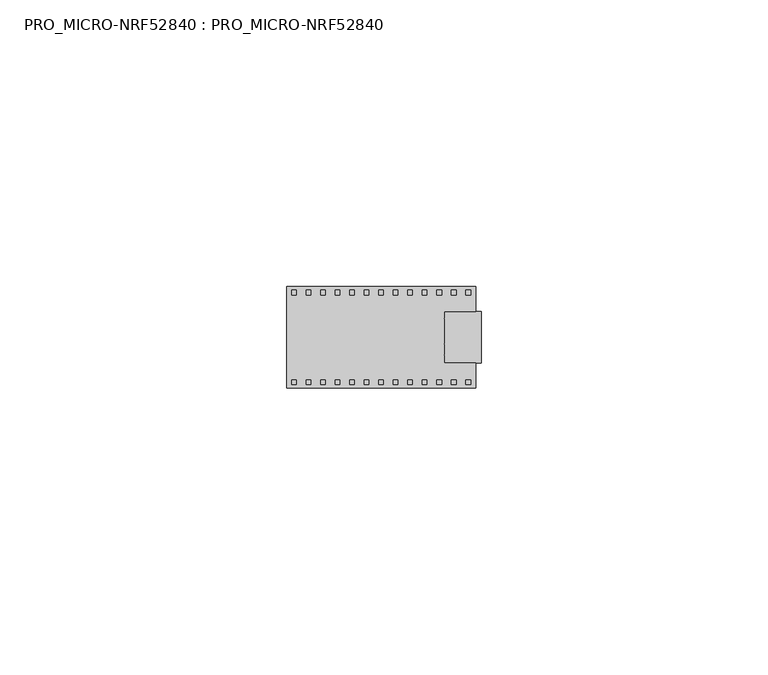
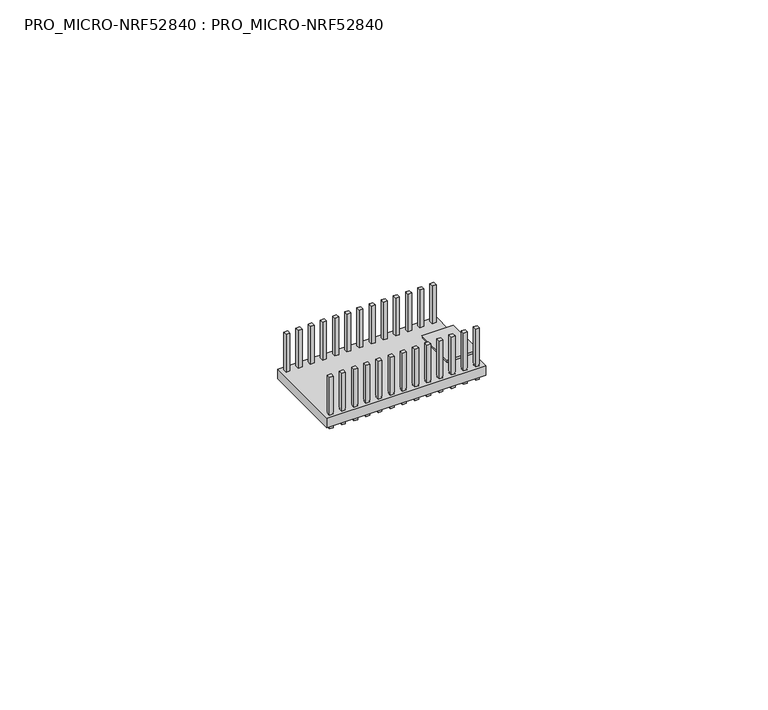
"""IFC4 building model written with IfcOpenShell, lengths in millimetres: furniture geometry, PRO_MICRO-NRF52840 : PRO_MICRO-NRF52840."""

from ifc_helpers import new_model, si_unit, origin, place, context, project, spatial, faceted_brep, source, transform, mapped, element, save


def pro_micro_nrf52840_pro_micro_nrf52840_bcfd0b97(model_context):
    return source(origin(), model_context, "Body", "Brep", [
        faceted_brep([(-14.8, 8.2144911, 11.3), (-15.6, 8.2144911, 11.3), (-15.6, 7.4144911, 11.3), (-14.8, 7.4144911, 11.3), (15.6, 8.2144911, 11.3), (14.8, 8.2144911, 11.3), (14.8, 7.4144911, 11.3), (15.6, 7.4144911, 11.3), (13.0666667, 8.2144911, 11.3), (12.2666667, 8.2144911, 11.3), (12.2666667, 7.4144911, 11.3), (13.0666667, 7.4144911, 11.3), (10.5333333, 8.2144911, 11.3), (9.7333333, 8.2144911, 11.3), (9.7333333, 7.4144911, 11.3), (10.5333333, 7.4144911, 11.3), (8.0, 8.2144911, 11.3), (7.2, 8.2144911, 11.3), (7.2, 7.4144911, 11.3), (8.0, 7.4144911, 11.3), (5.4666667, 8.2144911, 11.3), (4.6666667, 8.2144911, 11.3), (4.6666667, 7.4144911, 11.3), (5.4666667, 7.4144911, 11.3), (2.9333333, 8.2144911, 11.3), (2.1333333, 8.2144911, 11.3), (2.1333333, 7.4144911, 11.3), (2.9333333, 7.4144911, 11.3), (0.4, 8.2144911, 11.3), (-0.4, 8.2144911, 11.3), (-0.4, 7.4144911, 11.3), (0.4, 7.4144911, 11.3), (-2.1333333, 8.2144911, 11.3), (-2.9333333, 8.2144911, 11.3), (-2.9333333, 7.4144911, 11.3), (-2.1333333, 7.4144911, 11.3), (-4.6666667, 8.2144911, 11.3), (-5.4666667, 8.2144911, 11.3), (-5.4666667, 7.4144911, 11.3), (-4.6666667, 7.4144911, 11.3), (-7.2, 8.2144911, 11.3), (-8.0, 8.2144911, 11.3), (-8.0, 7.4144911, 11.3), (-7.2, 7.4144911, 11.3), (-9.7333333, 8.2144911, 11.3), (-10.5333333, 8.2144911, 11.3), (-10.5333333, 7.4144911, 11.3), (-9.7333333, 7.4144911, 11.3), (-12.2666667, 8.2144911, 11.3), (-13.0666667, 8.2144911, 11.3), (-13.0666667, 7.4144911, 11.3), (-12.2666667, 7.4144911, 11.3), (-14.8, 8.2144911, 0.0), (-14.8, 7.4144911, 0.0), (-15.6, 7.4144911, 0.0), (-15.6, 8.2144911, 0.0), (15.6, 8.2144911, 0.0), (15.6, 7.4144911, 0.0), (14.8, 7.4144911, 0.0), (14.8, 8.2144911, 0.0), (13.0666667, 8.2144911, 0.0), (13.0666667, 7.4144911, 0.0), (12.2666667, 7.4144911, 0.0), (12.2666667, 8.2144911, 0.0), (10.5333333, 8.2144911, 0.0), (10.5333333, 7.4144911, 0.0), (9.7333333, 7.4144911, 0.0), (9.7333333, 8.2144911, 0.0), (8.0, 8.2144911, 0.0), (8.0, 7.4144911, 0.0), (7.2, 7.4144911, 0.0), (7.2, 8.2144911, 0.0), (5.4666667, 8.2144911, 0.0), (5.4666667, 7.4144911, 0.0), (4.6666667, 7.4144911, 0.0), (4.6666667, 8.2144911, 0.0), (2.9333333, 8.2144911, 0.0), (2.9333333, 7.4144911, 0.0), (2.1333333, 7.4144911, 0.0), (2.1333333, 8.2144911, 0.0), (0.4, 8.2144911, 0.0), (0.4, 7.4144911, 0.0), (-0.4, 7.4144911, 0.0), (-0.4, 8.2144911, 0.0), (-2.1333333, 8.2144911, 0.0), (-2.1333333, 7.4144911, 0.0), (-2.9333333, 7.4144911, 0.0), (-2.9333333, 8.2144911, 0.0), (-4.6666667, 8.2144911, 0.0), (-4.6666667, 7.4144911, 0.0), (-5.4666667, 7.4144911, 0.0), (-5.4666667, 8.2144911, 0.0), (-7.2, 8.2144911, 0.0), (-7.2, 7.4144911, 0.0), (-8.0, 7.4144911, 0.0), (-8.0, 8.2144911, 0.0), (-9.7333333, 8.2144911, 0.0), (-9.7333333, 7.4144911, 0.0), (-10.5333333, 7.4144911, 0.0), (-10.5333333, 8.2144911, 0.0), (-12.2666667, 8.2144911, 0.0), (-12.2666667, 7.4144911, 0.0), (-13.0666667, 7.4144911, 0.0), (-13.0666667, 8.2144911, 0.0), (-14.8, 8.2144911, 3.0), (-15.6, 8.2144911, 3.0), (-15.6, 8.2144911, 1.0), (-14.8, 8.2144911, 1.0), (-15.6, 7.4144911, 3.0), (-15.6, 7.4144911, 1.0), (-14.8, 7.4144911, 3.0), (-14.8, 7.4144911, 1.0), (15.6, 8.2144911, 3.0), (14.8, 8.2144911, 3.0), (14.8, 8.2144911, 1.0), (15.6, 8.2144911, 1.0), (14.8, 7.4144911, 3.0), (14.8, 7.4144911, 1.0), (15.6, 7.4144911, 3.0), (15.6, 7.4144911, 1.0), (13.0666667, 8.2144911, 3.0), (12.2666667, 8.2144911, 3.0), (12.2666667, 8.2144911, 1.0), (13.0666667, 8.2144911, 1.0), (12.2666667, 7.4144911, 3.0), (12.2666667, 7.4144911, 1.0), (13.0666667, 7.4144911, 3.0), (13.0666667, 7.4144911, 1.0), (10.5333333, 8.2144911, 3.0), (9.7333333, 8.2144911, 3.0), (9.7333333, 8.2144911, 1.0), (10.5333333, 8.2144911, 1.0), (9.7333333, 7.4144911, 3.0), (9.7333333, 7.4144911, 1.0), (10.5333333, 7.4144911, 3.0), (10.5333333, 7.4144911, 1.0), (8.0, 8.2144911, 3.0), (7.2, 8.2144911, 3.0), (7.2, 8.2144911, 1.0), (8.0, 8.2144911, 1.0), (7.2, 7.4144911, 3.0), (7.2, 7.4144911, 1.0), (8.0, 7.4144911, 3.0), (8.0, 7.4144911, 1.0), (5.4666667, 8.2144911, 3.0), (4.6666667, 8.2144911, 3.0), (4.6666667, 8.2144911, 1.0), (5.4666667, 8.2144911, 1.0), (4.6666667, 7.4144911, 3.0), (4.6666667, 7.4144911, 1.0), (5.4666667, 7.4144911, 3.0), (5.4666667, 7.4144911, 1.0), (2.9333333, 8.2144911, 3.0), (2.1333333, 8.2144911, 3.0), (2.1333333, 8.2144911, 1.0), (2.9333333, 8.2144911, 1.0), (2.1333333, 7.4144911, 3.0), (2.1333333, 7.4144911, 1.0), (2.9333333, 7.4144911, 3.0), (2.9333333, 7.4144911, 1.0), (0.4, 8.2144911, 3.0), (-0.4, 8.2144911, 3.0), (-0.4, 8.2144911, 1.0), (0.4, 8.2144911, 1.0), (-0.4, 7.4144911, 3.0), (-0.4, 7.4144911, 1.0), (0.4, 7.4144911, 3.0), (0.4, 7.4144911, 1.0), (-2.1333333, 8.2144911, 3.0), (-2.9333333, 8.2144911, 3.0), (-2.9333333, 8.2144911, 1.0), (-2.1333333, 8.2144911, 1.0), (-2.9333333, 7.4144911, 3.0), (-2.9333333, 7.4144911, 1.0), (-2.1333333, 7.4144911, 3.0), (-2.1333333, 7.4144911, 1.0), (-4.6666667, 8.2144911, 3.0), (-5.4666667, 8.2144911, 3.0), (-5.4666667, 8.2144911, 1.0), (-4.6666667, 8.2144911, 1.0), (-5.4666667, 7.4144911, 3.0), (-5.4666667, 7.4144911, 1.0), (-4.6666667, 7.4144911, 3.0), (-4.6666667, 7.4144911, 1.0), (-7.2, 8.2144911, 3.0), (-8.0, 8.2144911, 3.0), (-8.0, 8.2144911, 1.0), (-7.2, 8.2144911, 1.0), (-8.0, 7.4144911, 3.0), (-8.0, 7.4144911, 1.0), (-7.2, 7.4144911, 3.0), (-7.2, 7.4144911, 1.0), (-9.7333333, 8.2144911, 3.0), (-10.5333333, 8.2144911, 3.0), (-10.5333333, 8.2144911, 1.0), (-9.7333333, 8.2144911, 1.0), (-10.5333333, 7.4144911, 3.0), (-10.5333333, 7.4144911, 1.0), (-9.7333333, 7.4144911, 3.0), (-9.7333333, 7.4144911, 1.0), (-12.2666667, 8.2144911, 3.0), (-13.0666667, 8.2144911, 3.0), (-13.0666667, 8.2144911, 1.0), (-12.2666667, 8.2144911, 1.0), (-13.0666667, 7.4144911, 3.0), (-13.0666667, 7.4144911, 1.0), (-12.2666667, 7.4144911, 3.0), (-12.2666667, 7.4144911, 1.0), (16.5, 8.89, 3.0), (-16.5, 8.89, 3.0), (-16.5, -8.89, 3.0), (16.5, -8.89, 3.0), (16.5, -4.5, 3.0), (11.0, -4.5, 3.0), (11.0, 4.5, 3.0), (16.5, 4.5, 3.0), (-14.8, -8.2144911, 3.0), (-15.6, -8.2144911, 3.0), (-15.6, -7.4144911, 3.0), (-14.8, -7.4144911, 3.0), (15.6, -8.2144911, 3.0), (14.8, -8.2144911, 3.0), (14.8, -7.4144911, 3.0), (15.6, -7.4144911, 3.0), (13.0666667, -8.2144911, 3.0), (12.2666667, -8.2144911, 3.0), (12.2666667, -7.4144911, 3.0), (13.0666667, -7.4144911, 3.0), (10.5333333, -8.2144911, 3.0), (9.7333333, -8.2144911, 3.0), (9.7333333, -7.4144911, 3.0), (10.5333333, -7.4144911, 3.0), (8.0, -8.2144911, 3.0), (7.2, -8.2144911, 3.0), (7.2, -7.4144911, 3.0), (8.0, -7.4144911, 3.0), (5.4666667, -8.2144911, 3.0), (4.6666667, -8.2144911, 3.0), (4.6666667, -7.4144911, 3.0), (5.4666667, -7.4144911, 3.0), (2.9333333, -8.2144911, 3.0), (2.1333333, -8.2144911, 3.0), (2.1333333, -7.4144911, 3.0), (2.9333333, -7.4144911, 3.0), (0.4, -8.2144911, 3.0), (-0.4, -8.2144911, 3.0), (-0.4, -7.4144911, 3.0), (0.4, -7.4144911, 3.0), (-2.1333333, -8.2144911, 3.0), (-2.9333333, -8.2144911, 3.0), (-2.9333333, -7.4144911, 3.0), (-2.1333333, -7.4144911, 3.0), (-4.6666667, -8.2144911, 3.0), (-5.4666667, -8.2144911, 3.0), (-5.4666667, -7.4144911, 3.0), (-4.6666667, -7.4144911, 3.0), (-7.2, -8.2144911, 3.0), (-8.0, -8.2144911, 3.0), (-8.0, -7.4144911, 3.0), (-7.2, -7.4144911, 3.0), (-9.7333333, -8.2144911, 3.0), (-10.5333333, -8.2144911, 3.0), (-10.5333333, -7.4144911, 3.0), (-9.7333333, -7.4144911, 3.0), (-12.2666667, -8.2144911, 3.0), (-13.0666667, -8.2144911, 3.0), (-13.0666667, -7.4144911, 3.0), (-12.2666667, -7.4144911, 3.0), (16.5, -8.89, 1.0), (-16.5, -8.89, 1.0), (-16.5, 8.89, 1.0), (16.5, 8.89, 1.0), (16.5, 4.5, 1.0), (11.0, 4.5, 1.0), (11.0, -4.5, 1.0), (16.5, -4.5, 1.0), (-15.6, -8.2144911, 1.0), (-14.8, -8.2144911, 1.0), (-14.8, -7.4144911, 1.0), (-15.6, -7.4144911, 1.0), (14.8, -8.2144911, 1.0), (15.6, -8.2144911, 1.0), (15.6, -7.4144911, 1.0), (14.8, -7.4144911, 1.0), (12.2666667, -8.2144911, 1.0), (13.0666667, -8.2144911, 1.0), (13.0666667, -7.4144911, 1.0), (12.2666667, -7.4144911, 1.0), (9.7333333, -8.2144911, 1.0), (10.5333333, -8.2144911, 1.0), (10.5333333, -7.4144911, 1.0), (9.7333333, -7.4144911, 1.0), (7.2, -8.2144911, 1.0), (8.0, -8.2144911, 1.0), (8.0, -7.4144911, 1.0), (7.2, -7.4144911, 1.0), (4.6666667, -8.2144911, 1.0), (5.4666667, -8.2144911, 1.0), (5.4666667, -7.4144911, 1.0), (4.6666667, -7.4144911, 1.0), (2.1333333, -8.2144911, 1.0), (2.9333333, -8.2144911, 1.0), (2.9333333, -7.4144911, 1.0), (2.1333333, -7.4144911, 1.0), (-0.4, -8.2144911, 1.0), (0.4, -8.2144911, 1.0), (0.4, -7.4144911, 1.0), (-0.4, -7.4144911, 1.0), (-2.9333333, -8.2144911, 1.0), (-2.1333333, -8.2144911, 1.0), (-2.1333333, -7.4144911, 1.0), (-2.9333333, -7.4144911, 1.0), (-5.4666667, -8.2144911, 1.0), (-4.6666667, -8.2144911, 1.0), (-4.6666667, -7.4144911, 1.0), (-5.4666667, -7.4144911, 1.0), (-8.0, -8.2144911, 1.0), (-7.2, -8.2144911, 1.0), (-7.2, -7.4144911, 1.0), (-8.0, -7.4144911, 1.0), (-10.5333333, -8.2144911, 1.0), (-9.7333333, -8.2144911, 1.0), (-9.7333333, -7.4144911, 1.0), (-10.5333333, -7.4144911, 1.0), (-13.0666667, -8.2144911, 1.0), (-12.2666667, -8.2144911, 1.0), (-12.2666667, -7.4144911, 1.0), (-13.0666667, -7.4144911, 1.0), (-14.8, -8.2144911, 11.3), (-14.8, -7.4144911, 11.3), (-15.6, -7.4144911, 11.3), (-15.6, -8.2144911, 11.3), (15.6, -8.2144911, 11.3), (15.6, -7.4144911, 11.3), (14.8, -7.4144911, 11.3), (14.8, -8.2144911, 11.3), (13.0666667, -8.2144911, 11.3), (13.0666667, -7.4144911, 11.3), (12.2666667, -7.4144911, 11.3), (12.2666667, -8.2144911, 11.3), (10.5333333, -8.2144911, 11.3), (10.5333333, -7.4144911, 11.3), (9.7333333, -7.4144911, 11.3), (9.7333333, -8.2144911, 11.3), (8.0, -8.2144911, 11.3), (8.0, -7.4144911, 11.3), (7.2, -7.4144911, 11.3), (7.2, -8.2144911, 11.3), (5.4666667, -8.2144911, 11.3), (5.4666667, -7.4144911, 11.3), (4.6666667, -7.4144911, 11.3), (4.6666667, -8.2144911, 11.3), (2.9333333, -8.2144911, 11.3), (2.9333333, -7.4144911, 11.3), (2.1333333, -7.4144911, 11.3), (2.1333333, -8.2144911, 11.3), (0.4, -8.2144911, 11.3), (0.4, -7.4144911, 11.3), (-0.4, -7.4144911, 11.3), (-0.4, -8.2144911, 11.3), (-2.1333333, -8.2144911, 11.3), (-2.1333333, -7.4144911, 11.3), (-2.9333333, -7.4144911, 11.3), (-2.9333333, -8.2144911, 11.3), (-4.6666667, -8.2144911, 11.3), (-4.6666667, -7.4144911, 11.3), (-5.4666667, -7.4144911, 11.3), (-5.4666667, -8.2144911, 11.3), (-7.2, -8.2144911, 11.3), (-7.2, -7.4144911, 11.3), (-8.0, -7.4144911, 11.3), (-8.0, -8.2144911, 11.3), (-9.7333333, -8.2144911, 11.3), (-9.7333333, -7.4144911, 11.3), (-10.5333333, -7.4144911, 11.3), (-10.5333333, -8.2144911, 11.3), (-12.2666667, -8.2144911, 11.3), (-12.2666667, -7.4144911, 11.3), (-13.0666667, -7.4144911, 11.3), (-13.0666667, -8.2144911, 11.3), (-14.8, -8.2144911, 0.0), (-15.6, -8.2144911, 0.0), (-15.6, -7.4144911, 0.0), (-14.8, -7.4144911, 0.0), (15.6, -8.2144911, 0.0), (14.8, -8.2144911, 0.0), (14.8, -7.4144911, 0.0), (15.6, -7.4144911, 0.0), (13.0666667, -8.2144911, 0.0), (12.2666667, -8.2144911, 0.0), (12.2666667, -7.4144911, 0.0), (13.0666667, -7.4144911, 0.0), (10.5333333, -8.2144911, 0.0), (9.7333333, -8.2144911, 0.0), (9.7333333, -7.4144911, 0.0), (10.5333333, -7.4144911, 0.0), (8.0, -8.2144911, 0.0), (7.2, -8.2144911, 0.0), (7.2, -7.4144911, 0.0), (8.0, -7.4144911, 0.0), (5.4666667, -8.2144911, 0.0), (4.6666667, -8.2144911, 0.0), (4.6666667, -7.4144911, 0.0), (5.4666667, -7.4144911, 0.0), (2.9333333, -8.2144911, 0.0), (2.1333333, -8.2144911, 0.0), (2.1333333, -7.4144911, 0.0), (2.9333333, -7.4144911, 0.0), (0.4, -8.2144911, 0.0), (-0.4, -8.2144911, 0.0), (-0.4, -7.4144911, 0.0), (0.4, -7.4144911, 0.0), (-2.1333333, -8.2144911, 0.0), (-2.9333333, -8.2144911, 0.0), (-2.9333333, -7.4144911, 0.0), (-2.1333333, -7.4144911, 0.0), (-4.6666667, -8.2144911, 0.0), (-5.4666667, -8.2144911, 0.0), (-5.4666667, -7.4144911, 0.0), (-4.6666667, -7.4144911, 0.0), (-7.2, -8.2144911, 0.0), (-8.0, -8.2144911, 0.0), (-8.0, -7.4144911, 0.0), (-7.2, -7.4144911, 0.0), (-9.7333333, -8.2144911, 0.0), (-10.5333333, -8.2144911, 0.0), (-10.5333333, -7.4144911, 0.0), (-9.7333333, -7.4144911, 0.0), (-12.2666667, -8.2144911, 0.0), (-13.0666667, -8.2144911, 0.0), (-13.0666667, -7.4144911, 0.0), (-12.2666667, -7.4144911, 0.0), (11.0, 4.5, 3.5), (11.0, -4.5, 3.5), (17.5, -4.5, 3.5), (17.5, 4.5, 3.5), (11.0, 4.5, 0.0), (17.5, 4.5, 0.0), (17.5, -4.5, 0.0), (11.0, -4.5, 0.0)], [[[0, 1, 2, 3]], [[4, 5, 6, 7]], [[8, 9, 10, 11]], [[12, 13, 14, 15]], [[16, 17, 18, 19]], [[20, 21, 22, 23]], [[24, 25, 26, 27]], [[28, 29, 30, 31]], [[32, 33, 34, 35]], [[36, 37, 38, 39]], [[40, 41, 42, 43]], [[44, 45, 46, 47]], [[48, 49, 50, 51]], [[52, 53, 54, 55]], [[56, 57, 58, 59]], [[60, 61, 62, 63]], [[64, 65, 66, 67]], [[68, 69, 70, 71]], [[72, 73, 74, 75]], [[76, 77, 78, 79]], [[80, 81, 82, 83]], [[84, 85, 86, 87]], [[88, 89, 90, 91]], [[92, 93, 94, 95]], [[96, 97, 98, 99]], [[100, 101, 102, 103]], [[1, 0, 104, 105]], [[52, 55, 106, 107]], [[2, 1, 105, 108]], [[55, 54, 109, 106]], [[3, 2, 108, 110]], [[54, 53, 111, 109]], [[0, 3, 110, 104]], [[53, 52, 107, 111]], [[5, 4, 112, 113]], [[56, 59, 114, 115]], [[6, 5, 113, 116]], [[59, 58, 117, 114]], [[7, 6, 116, 118]], [[58, 57, 119, 117]], [[4, 7, 118, 112]], [[57, 56, 115, 119]], [[9, 8, 120, 121]], [[60, 63, 122, 123]], [[10, 9, 121, 124]], [[63, 62, 125, 122]], [[11, 10, 124, 126]], [[62, 61, 127, 125]], [[8, 11, 126, 120]], [[61, 60, 123, 127]], [[13, 12, 128, 129]], [[64, 67, 130, 131]], [[14, 13, 129, 132]], [[67, 66, 133, 130]], [[15, 14, 132, 134]], [[66, 65, 135, 133]], [[12, 15, 134, 128]], [[65, 64, 131, 135]], [[17, 16, 136, 137]], [[68, 71, 138, 139]], [[18, 17, 137, 140]], [[71, 70, 141, 138]], [[19, 18, 140, 142]], [[70, 69, 143, 141]], [[16, 19, 142, 136]], [[69, 68, 139, 143]], [[21, 20, 144, 145]], [[72, 75, 146, 147]], [[22, 21, 145, 148]], [[75, 74, 149, 146]], [[23, 22, 148, 150]], [[74, 73, 151, 149]], [[20, 23, 150, 144]], [[73, 72, 147, 151]], [[25, 24, 152, 153]], [[76, 79, 154, 155]], [[26, 25, 153, 156]], [[79, 78, 157, 154]], [[27, 26, 156, 158]], [[78, 77, 159, 157]], [[24, 27, 158, 152]], [[77, 76, 155, 159]], [[29, 28, 160, 161]], [[80, 83, 162, 163]], [[30, 29, 161, 164]], [[83, 82, 165, 162]], [[31, 30, 164, 166]], [[82, 81, 167, 165]], [[28, 31, 166, 160]], [[81, 80, 163, 167]], [[33, 32, 168, 169]], [[84, 87, 170, 171]], [[34, 33, 169, 172]], [[87, 86, 173, 170]], [[35, 34, 172, 174]], [[86, 85, 175, 173]], [[32, 35, 174, 168]], [[85, 84, 171, 175]], [[37, 36, 176, 177]], [[88, 91, 178, 179]], [[38, 37, 177, 180]], [[91, 90, 181, 178]], [[39, 38, 180, 182]], [[90, 89, 183, 181]], [[36, 39, 182, 176]], [[89, 88, 179, 183]], [[41, 40, 184, 185]], [[92, 95, 186, 187]], [[42, 41, 185, 188]], [[95, 94, 189, 186]], [[43, 42, 188, 190]], [[94, 93, 191, 189]], [[40, 43, 190, 184]], [[93, 92, 187, 191]], [[45, 44, 192, 193]], [[96, 99, 194, 195]], [[46, 45, 193, 196]], [[99, 98, 197, 194]], [[47, 46, 196, 198]], [[98, 97, 199, 197]], [[44, 47, 198, 192]], [[97, 96, 195, 199]], [[49, 48, 200, 201]], [[100, 103, 202, 203]], [[50, 49, 201, 204]], [[103, 102, 205, 202]], [[51, 50, 204, 206]], [[102, 101, 207, 205]], [[48, 51, 206, 200]], [[101, 100, 203, 207]], [[208, 209, 210, 211, 212, 213, 214, 215], [105, 104, 110, 108], [113, 112, 118, 116], [121, 120, 126, 124], [129, 128, 134, 132], [137, 136, 142, 140], [145, 144, 150, 148], [153, 152, 158, 156], [161, 160, 166, 164], [169, 168, 174, 172], [177, 176, 182, 180], [185, 184, 190, 188], [193, 192, 198, 196], [201, 200, 206, 204], [216, 217, 218, 219], [220, 221, 222, 223], [224, 225, 226, 227], [228, 229, 230, 231], [232, 233, 234, 235], [236, 237, 238, 239], [240, 241, 242, 243], [244, 245, 246, 247], [248, 249, 250, 251], [252, 253, 254, 255], [256, 257, 258, 259], [260, 261, 262, 263], [264, 265, 266, 267]], [[268, 269, 270, 271, 272, 273, 274, 275], [107, 106, 109, 111], [115, 114, 117, 119], [123, 122, 125, 127], [131, 130, 133, 135], [139, 138, 141, 143], [147, 146, 149, 151], [155, 154, 157, 159], [163, 162, 165, 167], [171, 170, 173, 175], [179, 178, 181, 183], [187, 186, 189, 191], [195, 194, 197, 199], [203, 202, 205, 207], [276, 277, 278, 279], [280, 281, 282, 283], [284, 285, 286, 287], [288, 289, 290, 291], [292, 293, 294, 295], [296, 297, 298, 299], [300, 301, 302, 303], [304, 305, 306, 307], [308, 309, 310, 311], [312, 313, 314, 315], [316, 317, 318, 319], [320, 321, 322, 323], [324, 325, 326, 327]], [[209, 208, 271, 270]], [[210, 209, 270, 269]], [[211, 210, 269, 268]], [[271, 208, 215, 272]], [[211, 268, 275, 212]], [[328, 329, 330, 331]], [[332, 333, 334, 335]], [[336, 337, 338, 339]], [[340, 341, 342, 343]], [[344, 345, 346, 347]], [[348, 349, 350, 351]], [[352, 353, 354, 355]], [[356, 357, 358, 359]], [[360, 361, 362, 363]], [[364, 365, 366, 367]], [[368, 369, 370, 371]], [[372, 373, 374, 375]], [[376, 377, 378, 379]], [[380, 381, 382, 383]], [[384, 385, 386, 387]], [[388, 389, 390, 391]], [[392, 393, 394, 395]], [[396, 397, 398, 399]], [[400, 401, 402, 403]], [[404, 405, 406, 407]], [[408, 409, 410, 411]], [[412, 413, 414, 415]], [[416, 417, 418, 419]], [[420, 421, 422, 423]], [[424, 425, 426, 427]], [[428, 429, 430, 431]], [[328, 331, 217, 216]], [[381, 380, 277, 276]], [[331, 330, 218, 217]], [[382, 381, 276, 279]], [[330, 329, 219, 218]], [[383, 382, 279, 278]], [[329, 328, 216, 219]], [[380, 383, 278, 277]], [[332, 335, 221, 220]], [[385, 384, 281, 280]], [[335, 334, 222, 221]], [[386, 385, 280, 283]], [[334, 333, 223, 222]], [[387, 386, 283, 282]], [[333, 332, 220, 223]], [[384, 387, 282, 281]], [[336, 339, 225, 224]], [[389, 388, 285, 284]], [[339, 338, 226, 225]], [[390, 389, 284, 287]], [[338, 337, 227, 226]], [[391, 390, 287, 286]], [[337, 336, 224, 227]], [[388, 391, 286, 285]], [[340, 343, 229, 228]], [[393, 392, 289, 288]], [[343, 342, 230, 229]], [[394, 393, 288, 291]], [[342, 341, 231, 230]], [[395, 394, 291, 290]], [[341, 340, 228, 231]], [[392, 395, 290, 289]], [[344, 347, 233, 232]], [[397, 396, 293, 292]], [[347, 346, 234, 233]], [[398, 397, 292, 295]], [[346, 345, 235, 234]], [[399, 398, 295, 294]], [[345, 344, 232, 235]], [[396, 399, 294, 293]], [[348, 351, 237, 236]], [[401, 400, 297, 296]], [[351, 350, 238, 237]], [[402, 401, 296, 299]], [[350, 349, 239, 238]], [[403, 402, 299, 298]], [[349, 348, 236, 239]], [[400, 403, 298, 297]], [[352, 355, 241, 240]], [[405, 404, 301, 300]], [[355, 354, 242, 241]], [[406, 405, 300, 303]], [[354, 353, 243, 242]], [[407, 406, 303, 302]], [[353, 352, 240, 243]], [[404, 407, 302, 301]], [[356, 359, 245, 244]], [[409, 408, 305, 304]], [[359, 358, 246, 245]], [[410, 409, 304, 307]], [[358, 357, 247, 246]], [[411, 410, 307, 306]], [[357, 356, 244, 247]], [[408, 411, 306, 305]], [[360, 363, 249, 248]], [[413, 412, 309, 308]], [[363, 362, 250, 249]], [[414, 413, 308, 311]], [[362, 361, 251, 250]], [[415, 414, 311, 310]], [[361, 360, 248, 251]], [[412, 415, 310, 309]], [[364, 367, 253, 252]], [[417, 416, 313, 312]], [[367, 366, 254, 253]], [[418, 417, 312, 315]], [[366, 365, 255, 254]], [[419, 418, 315, 314]], [[365, 364, 252, 255]], [[416, 419, 314, 313]], [[368, 371, 257, 256]], [[421, 420, 317, 316]], [[371, 370, 258, 257]], [[422, 421, 316, 319]], [[370, 369, 259, 258]], [[423, 422, 319, 318]], [[369, 368, 256, 259]], [[420, 423, 318, 317]], [[372, 375, 261, 260]], [[425, 424, 321, 320]], [[375, 374, 262, 261]], [[426, 425, 320, 323]], [[374, 373, 263, 262]], [[427, 426, 323, 322]], [[373, 372, 260, 263]], [[424, 427, 322, 321]], [[376, 379, 265, 264]], [[429, 428, 325, 324]], [[379, 378, 266, 265]], [[430, 429, 324, 327]], [[378, 377, 267, 266]], [[431, 430, 327, 326]], [[377, 376, 264, 267]], [[428, 431, 326, 325]], [[432, 433, 434, 435]], [[436, 437, 438, 439]], [[433, 432, 214, 213]], [[436, 439, 274, 273]], [[434, 433, 213, 212, 275, 274, 439, 438]], [[435, 434, 438, 437]], [[432, 435, 437, 436, 273, 272, 215, 214]]]),
    ])


if __name__ == "__main__":
    model = new_model("IFC4")
    model_context = context("Model", 3, world=origin())
    ifc_project = project(units=[si_unit("LENGTHUNIT", "METRE", prefix="MILLI")], contexts=[model_context])
    site = spatial("IfcSite", under=ifc_project)
    building = spatial("IfcBuilding", under=site)
    placement = place(None, origin())
    pro_micro_nrf52840_pro_micro_nrf52840_shape = pro_micro_nrf52840_pro_micro_nrf52840_bcfd0b97(model_context)
    element("IfcFurniture", 1, ObjectType="PRO_MICRO-NRF52840 : PRO_MICRO-NRF52840", at=placement, inside=building, context=model_context, shape_type="MappedRepresentation", body=[
        mapped(pro_micro_nrf52840_pro_micro_nrf52840_shape, transform((0.0, 0.0, 0.0), x_axis=(1.0, 0.0, 0.0), y_axis=(0.0, 1.0, 0.0), z_axis=(0.0, 0.0, 1.0))),
    ])
    save(model, "model.ifc")

# Revit data of these elements
# Type "PRO_MICRO-NRF52840 : PRO_MICRO-NRF52840"
#   Default Elevation = 0
# Element 1 (IfcFurniture, "PRO_MICRO-NRF52840 : PRO_MICRO-NRF52840")
#   Materials on its faces: ".CHIP"
# Materials
#   ".CHIP": class "Vidro", colour RGB 236 240 239, transparency 0.35, Cost = 0
